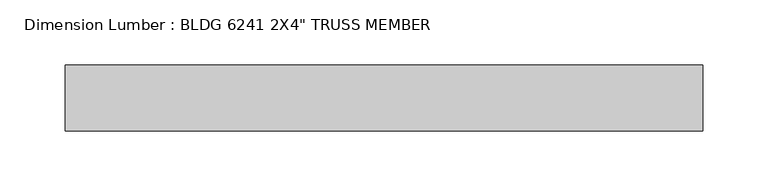
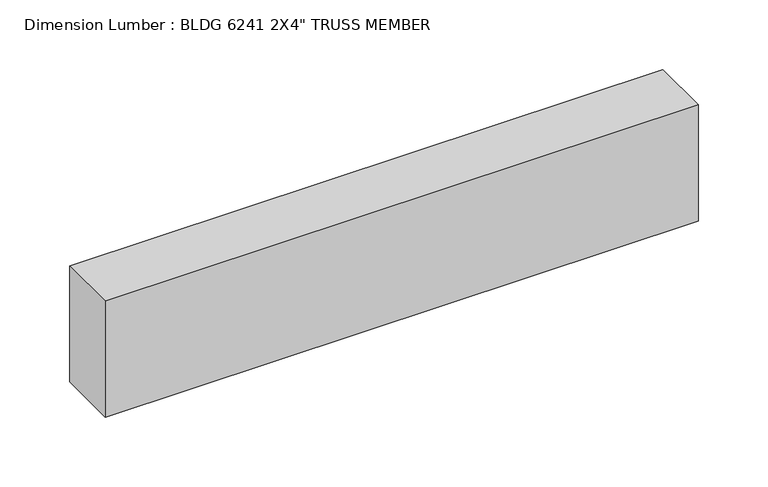
"""IFC4 building model written with IfcOpenShell, lengths in millimetres: beam geometry."""

from ifc_helpers import new_model, si_unit, frame, origin, place, context, project, spatial, polyline, outline, extrude, source, transform, mapped, element, save


def beam_42a29ae5(model_context):
    return source(origin(), model_context, "Body", "SweptSolid", [
        extrude(outline(polyline([(270.7395597, -25.4), (-219.9395597, -25.4), (-219.9395597, 25.4), (270.7395597, 25.4), (270.7395597, -25.4)])), frame((0.0, 0.0, -50.8), z_axis=(0.0, 0.0, 1.0), x_axis=(1.0, 0.0, 0.0)), (0.0, 0.0, 1.0), 101.6),
    ])


if __name__ == "__main__":
    model = new_model("IFC4")
    model_context = context("Model", 3, world=origin())
    ifc_project = project(units=[si_unit("LENGTHUNIT", "METRE", prefix="MILLI")], contexts=[model_context])
    site = spatial("IfcSite", under=ifc_project)
    building = spatial("IfcBuilding", under=site)
    placement = place(None, origin())
    beam_shape = beam_42a29ae5(model_context)
    element("IfcBeam", 1, ObjectType="Dimension Lumber : BLDG 6241 2X4\" TRUSS MEMBER", at=placement, inside=building, context=model_context, shape_type="MappedRepresentation", body=[
        mapped(beam_shape, transform((0.0, 0.0, 0.0), x_axis=(1.0, 0.0, 0.0), y_axis=(0.0, 1.0, 0.0), z_axis=(0.0, 0.0, 1.0))),
    ])
    save(model, "model.ifc")

# Revit data of these elements
# Type "Dimension Lumber : BLDG 6241 2X4\" TRUSS MEMBER"
#   Assembly Code = "B10"
#   A = 0.273472 SF
#   Length [instance default] = 5' - 0"
#   b = 0' - 2"
#   d = 0' - 4"
#   Structural Material [instance default] = Softwood, Lumber
# Element 1 (IfcBeam, "Dimension Lumber : BLDG 6241 2X4\" TRUSS MEMBER")
#   Materials on its faces: "Softwood, Lumber"
# Materials
#   "Softwood, Lumber": class "Wood", colour RGB 223 192 134, transparency 0, Description = "Pinus Echinata", Cost = 0
